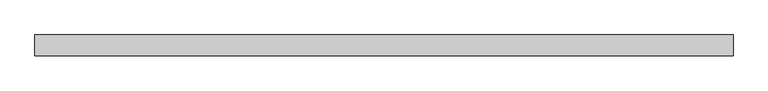
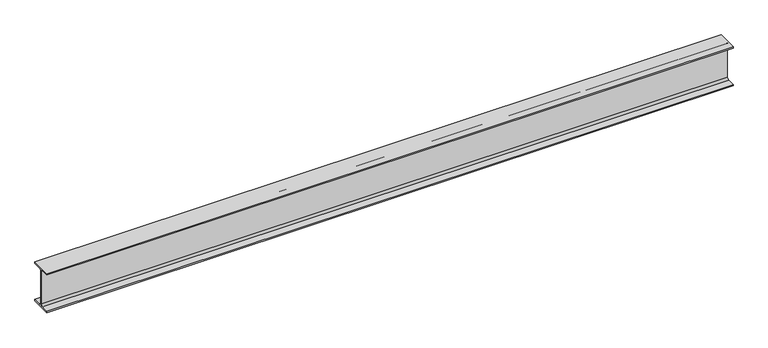
"""IFC4 building model written with IfcOpenShell, lengths in millimetres: beam geometry, 0912_Steel Framing_H-KSD3502 : H_SB_ASB_H-250x125x6x9."""

from ifc_helpers import new_model, si_unit, point, frame, frame_2d, origin, place, context, project, spatial, polyline, circle_curve, trimmed, segment, composite_curve, outline, extrude, source, transform, mapped, element, save


def beam_e15d8488(model_context):
    return source(origin(), model_context, "Body", "SweptSolid", [
        extrude(outline(composite_curve([segment(polyline([(62.5, -116.0), (62.5, -125.0), (-62.5, -125.0), (-62.5, -116.0), (-15.0, -116.0)]), True, "CONTINUOUS"), segment(trimmed(circle_curve(frame_2d((-15.0, -104.0)), 12.0), [point((-15.0, -116.0))], [point((-3.0, -104.0))], True, "CARTESIAN"), True, "CONTINUOUS"), segment(polyline([(-3.0, -104.0), (-3.0, 104.0)]), True, "CONTINUOUS"), segment(trimmed(circle_curve(frame_2d((-15.0, 104.0)), 12.0), [point((-3.0, 104.0))], [point((-15.0, 116.0))], True, "CARTESIAN"), True, "CONTINUOUS"), segment(polyline([(-15.0, 116.0), (-62.5, 116.0), (-62.5, 125.0), (62.5, 125.0), (62.5, 116.0), (15.0, 116.0)]), True, "CONTINUOUS"), segment(trimmed(circle_curve(frame_2d((15.0, 104.0)), 12.0), [point((15.0, 116.0))], [point((3.0, 104.0))], True, "CARTESIAN"), True, "CONTINUOUS"), segment(polyline([(3.0, 104.0), (3.0, -104.0)]), True, "CONTINUOUS"), segment(trimmed(circle_curve(frame_2d((15.0, -104.0)), 12.0), [point((3.0, -104.0))], [point((15.0, -116.0))], True, "CARTESIAN"), True, "CONTINUOUS"), segment(polyline([(15.0, -116.0), (62.5, -116.0)]), True, "CONTINUOUS")], self_intersect=False)), frame((-2029.8, 0.0, 0.0), z_axis=(1.0, 0.0, 0.0), x_axis=(0.0, 1.0, 0.0)), (0.0, 0.0, 1.0), 4142.0999994),
    ])


if __name__ == "__main__":
    model = new_model("IFC4")
    model_context = context("Model", 3, world=origin())
    ifc_project = project(units=[si_unit("LENGTHUNIT", "METRE", prefix="MILLI")], contexts=[model_context])
    site = spatial("IfcSite", under=ifc_project)
    building = spatial("IfcBuilding", under=site)
    placement = place(None, origin())
    beam_shape = beam_e15d8488(model_context)
    element("IfcBeam", 1, ObjectType="0912_Steel Framing_H-KSD3502 : H_SB_ASB_H-250x125x6x9", at=placement, inside=building, context=model_context, shape_type="MappedRepresentation", body=[
        mapped(beam_shape, transform((0.0, 0.0, 0.0), x_axis=(1.0, 0.0, 0.0), y_axis=(0.0, 1.0, 0.0), z_axis=(0.0, 0.0, 1.0))),
    ])
    save(model, "model.ifc")

# Revit data of these elements
# Type "0912_Steel Framing_H-KSD3502 : H_SB_ASB_H-250x125x6x9"
#   H_WM Code_1 = "S01AA003-00001 | Main Steel Structure Fabrication Work | Shelter/Building | Light Steel - Standard (30KG/M>Weight) | Material: (   )"
#   H_WM Code_2 = "S03AA029-00001 | Main Steel Structure Erection Work | Shelter/Building | Light Steel (30KG/M>Weight) | Material: (   )"
#   H_WM Code_3 = "S01AA010-00001 | Main Steel Structure Fabrication Work | Shelter/Building | Steel Painting/Coating | for Non-Fireproofed Steel Surface, Surface Preparation, Primer, Second & Final Coat | Material: (   )"
#   H_Q'ty Cal Type Tag = "SB-Q2"
#   Width = 12.5 cm
#   Web Thickness = 0.6 cm
#   Web Fillet = 1.2 cm
#   Warping Constant = 42539.8 cm⁶
#   W = 0
#   Torsional Moment of Inertia = 7.8102 cm⁴
#   Section Area = 37.66 cm²
#   Plastic Modulus weak axis = 73.1 cm³
#   Plastic Modulus strong axis = 366.0 cm³
#   Perimeter = 0.97 m²/m
#   Nominal Weight = 29.60 kgf/m
#   Moment of Inertia weak axis = 294.00 cm⁴
#   Moment of Inertia strong axis = 4050.00 cm⁴
#   Height = 25.0 cm
#   Flange Thickness = 0.9 cm
#   Elastic Modulus weak axis = 47.0 cm³
#   Elastic Modulus strong axis = 324.0 cm³
#   Centroid Vertical = 12.5 cm
#   Centroid Horizontal = 6.25 cm
#   Ix = 40500000
#   Length [instance default] = 1.5240 m
#   Zx = 366000
#   b = 0.1250 m
#   h = 0.2500 m
#   r = 0.0120 m
#   s = 0.0060 m
#   t = 0.0090 m
#   A = 0.003766 m²
#   Structural Material [instance default] = Steel, 45-345
#   Assembly Code = ""
# Element 1 (IfcBeam, "0912_Steel Framing_H-KSD3502 : H_SB_ASB_H-250x125x6x9")
#   Structural Material = none
# Materials
#   "Steel, 45-345": class "Metal", colour RGB 189 187 185, transparency 0, Description = "Steel 345 MPa", Cost = 0
